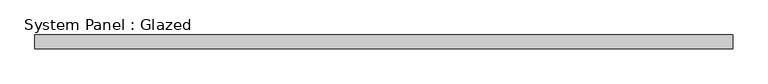
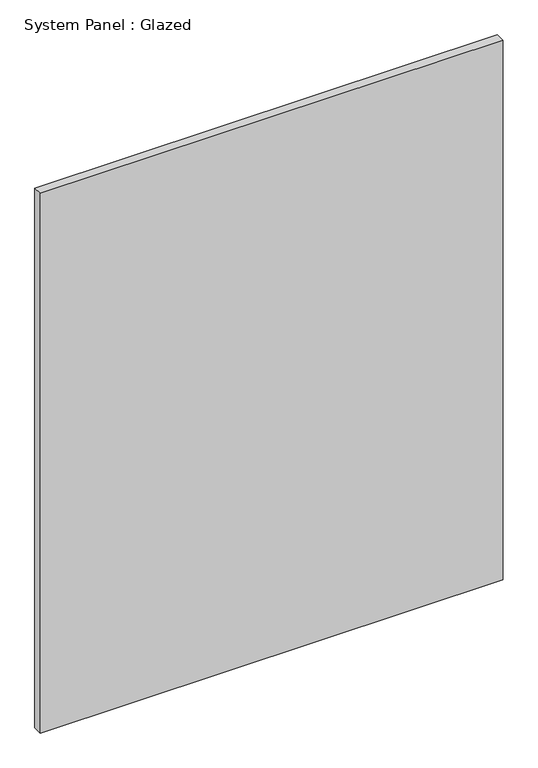
"""IFC4 building model written with IfcOpenShell, lengths in millimetres: plate geometry, System Panel : Glazed."""

import ifcopenshell
import ifcopenshell.guid

model = None  # the IFC model being written
_history = None  # IfcOwnerHistory: only IFC2X3 demands one
_inside = {}  # id of a spatial element -> (the spatial element, [elements in it])
_under = {}  # id of a project, library or spatial element -> (it, [spatial elements below it])
_declared = {}  # id of a project -> (the project, [libraries it declares])
_typed = {}  # id of a type object -> (the type object, [elements of that type])
_made_of = {}  # id of a material, layer set ... -> (it, [elements and type objects made of it])


def new_model(schema):
    """Start an empty IFC model of exactly this schema.

    Asked for "IFC4X3", IfcOpenShell would pick the latest addendum, in which some entities
    have other attributes; the version numbers below select the first issue.
    IFC2X3 requires an IfcOwnerHistory on every rooted entity: one is made here for all.
    """
    global model, _history
    if schema == "IFC4X3":
        model = ifcopenshell.file(schema_version=(4, 3, 0, 0))
    else:
        model = ifcopenshell.file(schema=schema)
    _inside.clear()
    _under.clear()
    _declared.clear()
    _typed.clear()
    _made_of.clear()
    _history = None
    if model.schema == "IFC2X3":
        org = make("IfcOrganization", Name="unknown")
        user = make(
            "IfcPersonAndOrganization",
            ThePerson=make("IfcPerson", FamilyName="unknown"),
            TheOrganization=org,
        )
        app = make(
            "IfcApplication",
            ApplicationDeveloper=org,
            Version="unknown",
            ApplicationFullName="unknown",
            ApplicationIdentifier="unknown",
        )
        _history = make(
            "IfcOwnerHistory",
            OwningUser=user,
            OwningApplication=app,
            ChangeAction="ADDED",
            CreationDate=0,
        )
    return model


def make(cls, **values):
    """One entity of the class cls with the attributes given. An attribute that is None is left unset."""
    return model.create_entity(
        cls, **{name: value for name, value in values.items() if value is not None}
    )


def rooted(cls, **values):
    """An entity with a GlobalId (a new one), such as an element, a storey or a relation."""
    return make(cls, GlobalId=ifcopenshell.guid.new(), OwnerHistory=_history, **values)


def si_unit(unit_type, name, prefix=None):
    """IfcSIUnit, for example si_unit("LENGTHUNIT", "METRE", prefix="MILLI")."""
    return make("IfcSIUnit", UnitType=unit_type, Prefix=prefix, Name=name)


def assignment(units):
    """IfcUnitAssignment: the units of a project."""
    return None if units is None else make("IfcUnitAssignment", Units=units)


def point(xyz):
    """IfcCartesianPoint."""
    return None if xyz is None else make("IfcCartesianPoint", Coordinates=xyz)


def direction(xyz):
    """IfcDirection."""
    return None if xyz is None else make("IfcDirection", DirectionRatios=xyz)


def frame(location, z_axis=None, x_axis=None):
    """IfcAxis2Placement3D, a coordinate frame: its origin and axes. An axis left out is left unset."""
    return make(
        "IfcAxis2Placement3D",
        Location=point(location),
        Axis=direction(z_axis),
        RefDirection=direction(x_axis),
    )


def origin():
    """The frame at (0, 0, 0) with its axes left unset."""
    return frame((0.0, 0.0, 0.0))


def origin_with_axes():
    """The frame at (0, 0, 0) with the z axis (0, 0, 1) and the x axis (1, 0, 0) written out."""
    return frame((0.0, 0.0, 0.0), z_axis=(0.0, 0.0, 1.0), x_axis=(1.0, 0.0, 0.0))


def place(relative_to, where):
    """IfcLocalPlacement: puts the frame where relative to a parent placement (None: the world)."""
    return make(
        "IfcLocalPlacement", PlacementRelTo=relative_to, RelativePlacement=where
    )


def context(
    kind, dimensions, precision=None, world=None, true_north=None, identifier=None
):
    """IfcGeometricRepresentationContext, for example the 3D "Model" context."""
    return make(
        "IfcGeometricRepresentationContext",
        ContextIdentifier=identifier,
        ContextType=kind,
        CoordinateSpaceDimension=dimensions,
        Precision=precision,
        WorldCoordinateSystem=world,
        TrueNorth=true_north,
    )


def project(units=None, contexts=None):
    """IfcProject with its units and contexts."""
    return rooted(
        "IfcProject",
        Name="project",
        RepresentationContexts=contexts,
        UnitsInContext=assignment(units),
    )


def spatial(cls, under=None, at=None, **own):
    """A site, building, storey or space (cls), placed at a placement, below another one or the project."""
    s = rooted(cls, ObjectPlacement=at, **own)
    if under is not None:
        _under.setdefault(under.id(), (under, []))[1].append(s)
    return s


def polyline(points):
    """IfcPolyline through the points."""
    return make("IfcPolyline", Points=[point(p) for p in points])


def outline(outer, holes=None, kind="AREA"):
    """IfcArbitraryClosedProfileDef: a profile drawn as a closed curve; with holes, ...WithVoids."""
    if holes is None:
        return make("IfcArbitraryClosedProfileDef", ProfileType=kind, OuterCurve=outer)
    return make(
        "IfcArbitraryProfileDefWithVoids",
        ProfileType=kind,
        OuterCurve=outer,
        InnerCurves=holes,
    )


def extrude(swept, where, along, depth):
    """IfcExtrudedAreaSolid: the profile swept, set in the frame where, extruded along a direction by depth."""
    return make(
        "IfcExtrudedAreaSolid",
        SweptArea=swept,
        Position=where,
        ExtrudedDirection=direction(along),
        Depth=depth,
    )


def shape(context_of_items, identifier, shape_type, items):
    """IfcShapeRepresentation: the items that make up one representation, for example the "Body"."""
    return make(
        "IfcShapeRepresentation",
        ContextOfItems=context_of_items,
        RepresentationIdentifier=identifier,
        RepresentationType=shape_type,
        Items=items,
    )


def source(mapping_origin, context_of_items, identifier, shape_type, items):
    """IfcRepresentationMap: a shape defined once, which mapped items show again and again."""
    return make(
        "IfcRepresentationMap",
        MappingOrigin=mapping_origin,
        MappedRepresentation=shape(context_of_items, identifier, shape_type, items),
    )


def transform(
    local_origin,
    x_axis=None,
    y_axis=None,
    z_axis=None,
    scale=None,
    scale2=None,
    scale3=None,
    uniform=True,
):
    """IfcCartesianTransformationOperator3D, or its non-uniform kind. x_axis, y_axis, z_axis: its Axis1, 2, 3."""
    if uniform:
        return make(
            "IfcCartesianTransformationOperator3D",
            Axis1=direction(x_axis),
            Axis2=direction(y_axis),
            LocalOrigin=point(local_origin),
            Scale=scale,
            Axis3=direction(z_axis),
        )
    return make(
        "IfcCartesianTransformationOperator3DnonUniform",
        Axis1=direction(x_axis),
        Axis2=direction(y_axis),
        LocalOrigin=point(local_origin),
        Scale=scale,
        Axis3=direction(z_axis),
        Scale2=scale2,
        Scale3=scale3,
    )


def mapped(mapping_source, mapping_target):
    """IfcMappedItem: shows the shape of a source again, moved by a transform."""
    return make(
        "IfcMappedItem", MappingSource=mapping_source, MappingTarget=mapping_target
    )


def made_of(thing, what):
    """Note that an element or type object is made of a material, layer set ...; save() writes the relation."""
    if what is not None:
        _made_of.setdefault(what.id(), (what, []))[1].append(thing)
    return thing


def element(
    cls,
    number,
    at=None,
    inside=None,
    cuts=None,
    type_object=None,
    material=None,
    context=None,
    identifier="Body",
    shape_type=None,
    held_by="IfcProductDefinitionShape",
    body=None,
    shapes=None,
    **own,
):
    """One element of the class cls, such as IfcWall. Its Tag is "e" and its number.

    at: its placement. inside: the storey or other place that contains it. cuts: it is an
    opening in that element (IfcRelVoidsElement). A single representation is given by context,
    identifier, shape_type and body (its items); several are given by shapes. held_by: the class
    of the entity that holds the representations. save() writes the other relations.
    """
    e = rooted(cls, Tag="e%d" % number, ObjectPlacement=at, **own)
    if body is not None:
        shapes = [shape(context, identifier, shape_type, body)]
    if shapes is not None:
        e.Representation = make(held_by, Representations=shapes)
    if inside is not None:
        _inside.setdefault(inside.id(), (inside, []))[1].append(e)
    if cuts is not None:
        rooted(
            "IfcRelVoidsElement", RelatingBuildingElement=cuts, RelatedOpeningElement=e
        )
    if type_object is not None:
        _typed.setdefault(type_object.id(), (type_object, []))[1].append(e)
    return made_of(e, material)


def aggregate(whole, parts):
    """IfcRelAggregates: a whole, such as a stair, and the parts it consists of."""
    return rooted("IfcRelAggregates", RelatingObject=whole, RelatedObjects=parts)


def save(model, path):
    """Write the relations noted so far, then the file.

    IfcRelAggregates (storeys below a building ...), IfcRelContainedInSpatialStructure (elements
    in a storey), IfcRelDefinesByType, IfcRelAssociatesMaterial and IfcRelDeclares: one each for
    every whole, place, type object, material and project.
    """
    for whole, parts in _under.values():
        aggregate(whole, parts)
    for where, things in _inside.values():
        rooted(
            "IfcRelContainedInSpatialStructure",
            RelatedElements=things,
            RelatingStructure=where,
        )
    for kind, things in _typed.values():
        rooted("IfcRelDefinesByType", RelatedObjects=things, RelatingType=kind)
    for what, things in _made_of.values():
        rooted("IfcRelAssociatesMaterial", RelatedObjects=things, RelatingMaterial=what)
    for by, libraries in _declared.values():
        rooted("IfcRelDeclares", RelatingContext=by, RelatedDefinitions=libraries)
    model.write(path)


def system_panel_glazed_79b5039f(model_context):
    return source(origin(), model_context, "Body", "SweptSolid", [
        extrude(outline(polyline([(633.0541355, 24.5), (-633.0541355, 24.5), (-633.0541355, 49.5), (633.0541355, 49.5), (633.0541355, 24.5)])), origin_with_axes(), (0.0, 0.0, 1.0), 1560.0991456),
    ])


if __name__ == "__main__":
    model = new_model("IFC4")
    model_context = context("Model", 3, world=origin())
    ifc_project = project(units=[si_unit("LENGTHUNIT", "METRE", prefix="MILLI")], contexts=[model_context])
    site = spatial("IfcSite", under=ifc_project)
    building = spatial("IfcBuilding", under=site)
    placement = place(None, origin())
    system_panel_glazed_shape = system_panel_glazed_79b5039f(model_context)
    element("IfcPlate", 1, ObjectType="System Panel : Glazed", at=placement, inside=building, context=model_context, shape_type="MappedRepresentation", body=[
        mapped(system_panel_glazed_shape, transform((0.0, 0.0, 0.0), x_axis=(1.0, 0.0, 0.0), y_axis=(0.0, 1.0, 0.0), z_axis=(0.0, 0.0, 1.0))),
    ])
    save(model, "model.ifc")

# Revit data of these elements
# Type "System Panel : Glazed"
#   Construction Type Id = "GSP4R"
#   Analytic Construction = "1/8 in Pilkington single glazing"
#   Visual Light Transmittance = 0.9
#   Solar Heat Gain Coefficient = 0.86
#   Heat Transfer Coefficient (U) = 6.7069 W/(m²·K)
#   Define Thermal Properties by = 1
# Element 1 (IfcPlate, "System Panel : Glazed")
#   Materials on its faces: "Glass"
# Materials
#   "Glass": class "Glass", colour RGB 0 128 192, transparency 0.9, Description = "Soda Lime Glass", Cost = 0
